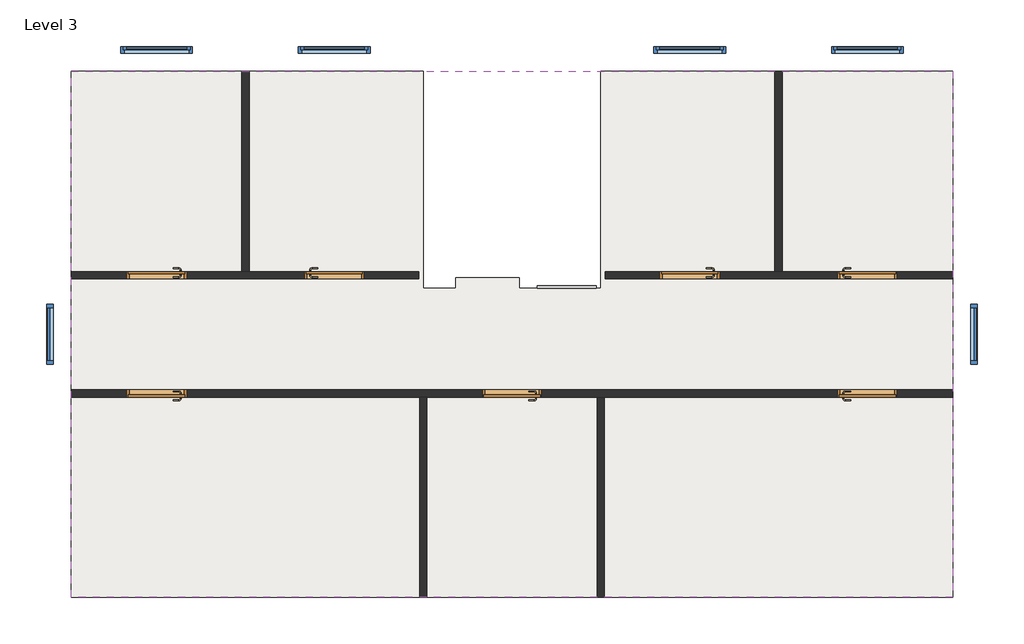
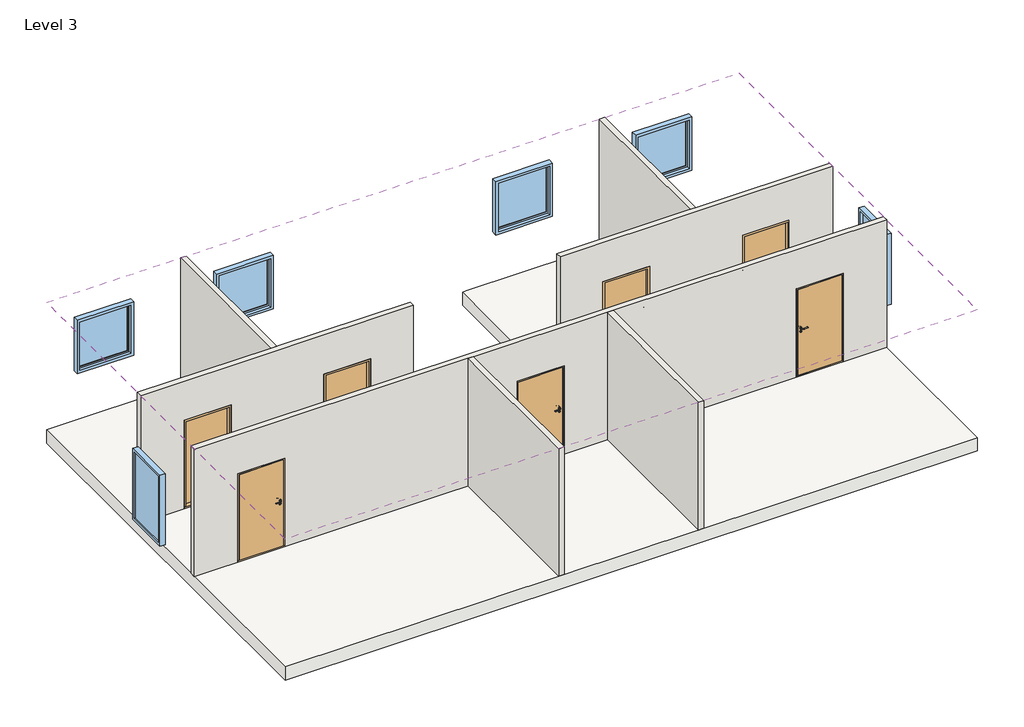
# One storey: 7 doors, 7 walls, 6 windows, 1 railing, 1 roof, 1 slab.
"""IFC4 building model written with IfcOpenShell, lengths in millimetres."""

import ifcopenshell
import ifcopenshell.guid

model = None  # the IFC model being written
_history = None  # IfcOwnerHistory: only IFC2X3 demands one
_inside = {}  # id of a spatial element -> (the spatial element, [elements in it])
_under = {}  # id of a project, library or spatial element -> (it, [spatial elements below it])
_declared = {}  # id of a project -> (the project, [libraries it declares])
_typed = {}  # id of a type object -> (the type object, [elements of that type])
_made_of = {}  # id of a material, layer set ... -> (it, [elements and type objects made of it])


def new_model(schema):
    """Start an empty IFC model of exactly this schema.

    Asked for "IFC4X3", IfcOpenShell would pick the latest addendum, in which some entities
    have other attributes; the version numbers below select the first issue.
    IFC2X3 requires an IfcOwnerHistory on every rooted entity: one is made here for all.
    """
    global model, _history
    if schema == "IFC4X3":
        model = ifcopenshell.file(schema_version=(4, 3, 0, 0))
    else:
        model = ifcopenshell.file(schema=schema)
    _inside.clear()
    _under.clear()
    _declared.clear()
    _typed.clear()
    _made_of.clear()
    _history = None
    if model.schema == "IFC2X3":
        org = make("IfcOrganization", Name="unknown")
        user = make(
            "IfcPersonAndOrganization",
            ThePerson=make("IfcPerson", FamilyName="unknown"),
            TheOrganization=org,
        )
        app = make(
            "IfcApplication",
            ApplicationDeveloper=org,
            Version="unknown",
            ApplicationFullName="unknown",
            ApplicationIdentifier="unknown",
        )
        _history = make(
            "IfcOwnerHistory",
            OwningUser=user,
            OwningApplication=app,
            ChangeAction="ADDED",
            CreationDate=0,
        )
    return model


def make(cls, **values):
    """One entity of the class cls with the attributes given. An attribute that is None is left unset."""
    return model.create_entity(
        cls, **{name: value for name, value in values.items() if value is not None}
    )


def rooted(cls, **values):
    """An entity with a GlobalId (a new one), such as an element, a storey or a relation."""
    return make(cls, GlobalId=ifcopenshell.guid.new(), OwnerHistory=_history, **values)


def si_unit(unit_type, name, prefix=None):
    """IfcSIUnit, for example si_unit("LENGTHUNIT", "METRE", prefix="MILLI")."""
    return make("IfcSIUnit", UnitType=unit_type, Prefix=prefix, Name=name)


def assignment(units):
    """IfcUnitAssignment: the units of a project."""
    return None if units is None else make("IfcUnitAssignment", Units=units)


def point(xyz):
    """IfcCartesianPoint."""
    return None if xyz is None else make("IfcCartesianPoint", Coordinates=xyz)


def direction(xyz):
    """IfcDirection."""
    return None if xyz is None else make("IfcDirection", DirectionRatios=xyz)


def frame(location, z_axis=None, x_axis=None):
    """IfcAxis2Placement3D, a coordinate frame: its origin and axes. An axis left out is left unset."""
    return make(
        "IfcAxis2Placement3D",
        Location=point(location),
        Axis=direction(z_axis),
        RefDirection=direction(x_axis),
    )


def frame_2d(location, x_axis=None):
    """IfcAxis2Placement2D, a coordinate frame in the plane: its origin and x axis."""
    return make(
        "IfcAxis2Placement2D", Location=point(location), RefDirection=direction(x_axis)
    )


def origin():
    """The frame at (0, 0, 0) with its axes left unset."""
    return frame((0.0, 0.0, 0.0))


def place(relative_to, where):
    """IfcLocalPlacement: puts the frame where relative to a parent placement (None: the world)."""
    return make(
        "IfcLocalPlacement", PlacementRelTo=relative_to, RelativePlacement=where
    )


def context(
    kind, dimensions, precision=None, world=None, true_north=None, identifier=None
):
    """IfcGeometricRepresentationContext, for example the 3D "Model" context."""
    return make(
        "IfcGeometricRepresentationContext",
        ContextIdentifier=identifier,
        ContextType=kind,
        CoordinateSpaceDimension=dimensions,
        Precision=precision,
        WorldCoordinateSystem=world,
        TrueNorth=true_north,
    )


def project(units=None, contexts=None):
    """IfcProject with its units and contexts."""
    return rooted(
        "IfcProject",
        Name="project",
        RepresentationContexts=contexts,
        UnitsInContext=assignment(units),
    )


def spatial(cls, under=None, at=None, **own):
    """A site, building, storey or space (cls), placed at a placement, below another one or the project."""
    s = rooted(cls, ObjectPlacement=at, **own)
    if under is not None:
        _under.setdefault(under.id(), (under, []))[1].append(s)
    return s


def polyline(points):
    """IfcPolyline through the points."""
    return make("IfcPolyline", Points=[point(p) for p in points])


def circle_curve(where, radius):
    """IfcCircle in the frame where."""
    return make("IfcCircle", Position=where, Radius=radius)


def ellipse_curve(where, semi_axis1, semi_axis2):
    """IfcEllipse in the frame where."""
    return make(
        "IfcEllipse", Position=where, SemiAxis1=semi_axis1, SemiAxis2=semi_axis2
    )


def trimmed(basis, trim1, trim2, sense, master):
    """IfcTrimmedCurve: the piece of a basis curve between two trims."""
    return make(
        "IfcTrimmedCurve",
        BasisCurve=basis,
        Trim1=trim1,
        Trim2=trim2,
        SenseAgreement=sense,
        MasterRepresentation=master,
    )


def segment(curve, same_sense, transition):
    """IfcCompositeCurveSegment."""
    return make(
        "IfcCompositeCurveSegment",
        Transition=transition,
        SameSense=same_sense,
        ParentCurve=curve,
    )


def composite_curve(segments, self_intersect=None):
    """IfcCompositeCurve: segments joined end to end."""
    return make("IfcCompositeCurve", Segments=segments, SelfIntersect=self_intersect)


def outline(outer, holes=None, kind="AREA"):
    """IfcArbitraryClosedProfileDef: a profile drawn as a closed curve; with holes, ...WithVoids."""
    if holes is None:
        return make("IfcArbitraryClosedProfileDef", ProfileType=kind, OuterCurve=outer)
    return make(
        "IfcArbitraryProfileDefWithVoids",
        ProfileType=kind,
        OuterCurve=outer,
        InnerCurves=holes,
    )


def extrude(swept, where, along, depth):
    """IfcExtrudedAreaSolid: the profile swept, set in the frame where, extruded along a direction by depth."""
    return make(
        "IfcExtrudedAreaSolid",
        SweptArea=swept,
        Position=where,
        ExtrudedDirection=direction(along),
        Depth=depth,
    )


def faces_of(points, faces, orient=None, outer=None):
    """IfcFace entities. A face is a list of loops; a loop is a list of indices into points, from 0.

    orient and outer hold one flag for each loop. By default every Orientation is true, the
    first loop of a face is its IfcFaceOuterBound and the others are IfcFaceBound.
    """
    made = []
    for i, loops in enumerate(faces):
        bounds = []
        for j, loop in enumerate(loops):
            is_outer = j == 0 if outer is None else outer[i][j]
            bounds.append(
                make(
                    "IfcFaceOuterBound" if is_outer else "IfcFaceBound",
                    Bound=make("IfcPolyLoop", Polygon=[points[k] for k in loop]),
                    Orientation=True if orient is None else orient[i][j],
                )
            )
        made.append(make("IfcFace", Bounds=bounds))
    return made


def faceted_brep(points, faces, orient=None, outer=None, voids=None):
    """IfcFacetedBrep: a solid bounded by flat faces; with voids (closed shells), ...WithVoids."""
    shared = [point(p) for p in points]
    hull = make("IfcClosedShell", CfsFaces=faces_of(shared, faces, orient, outer))
    if voids is None:
        return make("IfcFacetedBrep", Outer=hull)
    return make(
        "IfcFacetedBrepWithVoids",
        Outer=hull,
        Voids=[
            make(cls, CfsFaces=faces_of(shared, fs, o, b)) for cls, fs, o, b in voids
        ],
    )


def shape(context_of_items, identifier, shape_type, items):
    """IfcShapeRepresentation: the items that make up one representation, for example the "Body"."""
    return make(
        "IfcShapeRepresentation",
        ContextOfItems=context_of_items,
        RepresentationIdentifier=identifier,
        RepresentationType=shape_type,
        Items=items,
    )


def source(mapping_origin, context_of_items, identifier, shape_type, items):
    """IfcRepresentationMap: a shape defined once, which mapped items show again and again."""
    return make(
        "IfcRepresentationMap",
        MappingOrigin=mapping_origin,
        MappedRepresentation=shape(context_of_items, identifier, shape_type, items),
    )


def transform(
    local_origin,
    x_axis=None,
    y_axis=None,
    z_axis=None,
    scale=None,
    scale2=None,
    scale3=None,
    uniform=True,
):
    """IfcCartesianTransformationOperator3D, or its non-uniform kind. x_axis, y_axis, z_axis: its Axis1, 2, 3."""
    if uniform:
        return make(
            "IfcCartesianTransformationOperator3D",
            Axis1=direction(x_axis),
            Axis2=direction(y_axis),
            LocalOrigin=point(local_origin),
            Scale=scale,
            Axis3=direction(z_axis),
        )
    return make(
        "IfcCartesianTransformationOperator3DnonUniform",
        Axis1=direction(x_axis),
        Axis2=direction(y_axis),
        LocalOrigin=point(local_origin),
        Scale=scale,
        Axis3=direction(z_axis),
        Scale2=scale2,
        Scale3=scale3,
    )


def mapped(mapping_source, mapping_target):
    """IfcMappedItem: shows the shape of a source again, moved by a transform."""
    return make(
        "IfcMappedItem", MappingSource=mapping_source, MappingTarget=mapping_target
    )


def made_of(thing, what):
    """Note that an element or type object is made of a material, layer set ...; save() writes the relation."""
    if what is not None:
        _made_of.setdefault(what.id(), (what, []))[1].append(thing)
    return thing


def element(
    cls,
    number,
    at=None,
    inside=None,
    cuts=None,
    type_object=None,
    material=None,
    context=None,
    identifier="Body",
    shape_type=None,
    held_by="IfcProductDefinitionShape",
    body=None,
    shapes=None,
    **own,
):
    """One element of the class cls, such as IfcWall. Its Tag is "e" and its number.

    at: its placement. inside: the storey or other place that contains it. cuts: it is an
    opening in that element (IfcRelVoidsElement). A single representation is given by context,
    identifier, shape_type and body (its items); several are given by shapes. held_by: the class
    of the entity that holds the representations. save() writes the other relations.
    """
    e = rooted(cls, Tag="e%d" % number, ObjectPlacement=at, **own)
    if body is not None:
        shapes = [shape(context, identifier, shape_type, body)]
    if shapes is not None:
        e.Representation = make(held_by, Representations=shapes)
    if inside is not None:
        _inside.setdefault(inside.id(), (inside, []))[1].append(e)
    if cuts is not None:
        rooted(
            "IfcRelVoidsElement", RelatingBuildingElement=cuts, RelatedOpeningElement=e
        )
    if type_object is not None:
        _typed.setdefault(type_object.id(), (type_object, []))[1].append(e)
    return made_of(e, material)


def aggregate(whole, parts):
    """IfcRelAggregates: a whole, such as a stair, and the parts it consists of."""
    return rooted("IfcRelAggregates", RelatingObject=whole, RelatedObjects=parts)


def save(model, path):
    """Write the relations noted so far, then the file.

    IfcRelAggregates (storeys below a building ...), IfcRelContainedInSpatialStructure (elements
    in a storey), IfcRelDefinesByType, IfcRelAssociatesMaterial and IfcRelDeclares: one each for
    every whole, place, type object, material and project.
    """
    for whole, parts in _under.values():
        aggregate(whole, parts)
    for where, things in _inside.values():
        rooted(
            "IfcRelContainedInSpatialStructure",
            RelatedElements=things,
            RelatingStructure=where,
        )
    for kind, things in _typed.values():
        rooted("IfcRelDefinesByType", RelatedObjects=things, RelatingType=kind)
    for what, things in _made_of.values():
        rooted("IfcRelAssociatesMaterial", RelatedObjects=things, RelatingMaterial=what)
    for by, libraries in _declared.values():
        rooted("IfcRelDeclares", RelatingContext=by, RelatedDefinitions=libraries)
    model.write(path)


def plane_surface(at):
    """IfcPlane: the flat surface through the origin of the frame at, square to its z axis."""
    return make("IfcPlane", Position=at)


def cylinder_surface(at, radius):
    """IfcCylindricalSurface: all points at the distance radius from the z axis of the frame at."""
    return make("IfcCylindricalSurface", Position=at, Radius=radius)


def revolved_surface(curve, axis_point, axis_direction):
    """IfcSurfaceOfRevolution: the curve turned about the line through axis_point along axis_direction."""
    return make(
        "IfcSurfaceOfRevolution",
        SweptCurve=make("IfcArbitraryOpenProfileDef", ProfileType="CURVE", Curve=curve),
        AxisPosition=make("IfcAxis1Placement", Location=point(axis_point), Axis=direction(axis_direction)),
    )


def advanced_brep(points, edges, surfaces, faces):
    """IfcAdvancedBrep: a solid bounded by faces that lie on surfaces and meet in shared edges.

    An edge is (start, end): straight between two places in points (the first is 0);
    or (start, end, curve); or (start, end, curve, False) where it runs against its curve.
    A face is (place in surfaces, loops), or (place, loops, False) where it looks against
    its surface's normal. A loop lists edges by number (the first is 1), with a minus sign
    where the edge is run from its end to its start. The first loop is the outer one.
    """
    corners = [point(p) for p in points]
    vertices = [make("IfcVertexPoint", VertexGeometry=c) for c in corners]
    made = []
    for start, end, *more in edges:
        made.append(
            make(
                "IfcEdgeCurve",
                EdgeStart=vertices[start],
                EdgeEnd=vertices[end],
                EdgeGeometry=more[0] if more else make("IfcPolyline", Points=[corners[start], corners[end]]),
                SameSense=more[1] if len(more) > 1 else True,
            )
        )
    hull = []
    for where, loops, *sense in faces:
        bounds = []
        for j, loop in enumerate(loops):
            ring = [make("IfcOrientedEdge", EdgeElement=made[abs(k) - 1], Orientation=k > 0) for k in loop]
            bounds.append(
                make(
                    "IfcFaceOuterBound" if j == 0 else "IfcFaceBound",
                    Bound=make("IfcEdgeLoop", EdgeList=ring),
                    Orientation=True,
                )
            )
        hull.append(make("IfcAdvancedFace", Bounds=bounds, FaceSurface=surfaces[where], SameSense=sense[0] if sense else True))
    return make("IfcAdvancedBrep", Outer=make("IfcClosedShell", CfsFaces=hull))


def int_single_flush_10x20m_e84bf50b(model_context):
    return source(origin(), model_context, "Body", "SolidModel", [
        extrude(outline(composite_curve([segment(trimmed(circle_curve(frame_2d((1090.0, -406.0)), 20.0), [point((1070.0, -406.0))], [point((1110.0, -406.0))], False, "CARTESIAN"), True, "CONTINUOUS"), segment(trimmed(circle_curve(frame_2d((1090.0, -406.0)), 20.0), [point((1110.0, -406.0))], [point((1070.0, -406.0))], False, "CARTESIAN"), True, "CONTINUOUS")], self_intersect=False)), frame((0.0, 60.0, 0.0), z_axis=(0.0, 1.0, 0.0), x_axis=(0.0, 0.0, 1.0)), (0.0, 0.0, 1.0), 2.0),
        advanced_brep(
        [(-413.5, 62.0, 1090.0), (-398.5, 62.0, 1090.0), (-413.5, 84.5, 1090.0), (-398.5, 84.5, 1090.0), (-376.0, 107.0, 1090.0), (-376.0, 122.0, 1090.0), (-281.0, 122.0, 1090.0), (-281.0, 107.0, 1090.0)],
        [
            (0, 1, circle_curve(frame((-406.0, 62.0, 1090.0), z_axis=(0.0, -1.0, 0.0), x_axis=(1.0, 0.0, 0.0)), 7.5)),
            (1, 0, circle_curve(frame((-406.0, 62.0, 1090.0), z_axis=(0.0, -1.0, 0.0), x_axis=(1.0, 0.0, 0.0)), 7.5)),
            (0, 2),
            (2, 3, circle_curve(frame((-406.0, 84.5, 1090.0), z_axis=(0.0, -1.0, 0.0), x_axis=(1.0, 0.0, 0.0)), 7.5)),
            (3, 1),
            (3, 2, circle_curve(frame((-406.0, 84.5, 1090.0), z_axis=(0.0, -1.0, 0.0), x_axis=(1.0, 0.0, 0.0)), 7.5)),
            (4, 3, circle_curve(frame((-376.0, 84.5, 1090.0), z_axis=(0.0, 0.0, 1.0), x_axis=(-1.0, 0.0, 0.0)), 22.5)),
            (2, 5, circle_curve(frame((-376.0, 84.5, 1090.0), z_axis=(0.0, 0.0, -1.0), x_axis=(-1.0, 0.0, 0.0)), 37.5)),
            (5, 4, circle_curve(frame((-376.0, 114.5, 1090.0), z_axis=(-1.0, 0.0, 0.0), x_axis=(0.0, -1.0, 0.0)), 7.5)),
            (4, 5, circle_curve(frame((-376.0, 114.5, 1090.0), z_axis=(-1.0, 0.0, 0.0), x_axis=(0.0, -1.0, 0.0)), 7.5)),
            (5, 6),
            (6, 7, circle_curve(frame((-281.0, 114.5, 1090.0), z_axis=(-1.0, 0.0, 0.0), x_axis=(0.0, -1.0, 0.0)), 7.5)),
            (7, 4),
            (7, 6, circle_curve(frame((-281.0, 114.5, 1090.0), z_axis=(-1.0, 0.0, 0.0), x_axis=(0.0, -1.0, 0.0)), 7.5)),
        ],
        [
            plane_surface(frame((-406.0, 62.0, 1090.0), z_axis=(0.0, -1.0, 0.0), x_axis=(0.0, 0.0, -1.0))),
            cylinder_surface(frame((-406.0, 62.0, 1090.0), z_axis=(0.0, -1.0, 0.0), x_axis=(1.0, 0.0, 0.0)), 7.5),
            revolved_surface(trimmed(ellipse_curve(frame((-406.0, 84.5, 1090.0), z_axis=(0.0, -1.0, 0.0), x_axis=(1.0, 0.0, 0.0)), 7.5, 7.5), [point((-413.5, 84.5, 1090.0))], [point((-398.5, 84.5, 1090.0))], True, "CARTESIAN"), (-376.0, 84.5, 1090.0), (0.0, 0.0, -1.0)),
            revolved_surface(trimmed(ellipse_curve(frame((-406.0, 84.5, 1090.0), z_axis=(0.0, -1.0, 0.0), x_axis=(1.0, 0.0, 0.0)), 7.5, 7.5), [point((-398.5, 84.5, 1090.0))], [point((-413.5, 84.5, 1090.0))], True, "CARTESIAN"), (-376.0, 84.5, 1090.0), (0.0, 0.0, -1.0)),
            cylinder_surface(frame((-376.0, 114.5, 1090.0), z_axis=(-1.0, 0.0, 0.0), x_axis=(0.0, -1.0, 0.0)), 7.5),
            plane_surface(frame((-281.0, 114.5, 1090.0), z_axis=(1.0, 0.0, 0.0), x_axis=(0.0, 0.0, -1.0))),
        ],
        [
            (0, [[1, 2]]),
            (1, [[-1, 3, 4, 5]]),
            (1, [[-2, -5, 6, -3]]),
            (2, [[7, -4, 8, 9]]),
            (3, [[-8, -6, -7, 10]]),
            (4, [[-9, 11, 12, 13]]),
            (4, [[-10, -13, 14, -11]]),
            (5, [[-14, -12]]),
        ],
    ),
        extrude(outline(composite_curve([segment(trimmed(circle_curve(frame_2d((1010.0, -406.0)), 20.0), [point((990.0, -406.0))], [point((1030.0, -406.0))], False, "CARTESIAN"), True, "CONTINUOUS"), segment(trimmed(circle_curve(frame_2d((1010.0, -406.0)), 20.0), [point((1030.0, -406.0))], [point((990.0, -406.0))], False, "CARTESIAN"), True, "CONTINUOUS")], self_intersect=False), holes=[composite_curve([segment(trimmed(circle_curve(frame_2d((1015.0, -406.0)), 3.0), [point((1012.4019238, -407.5))], [point((1012.4019238, -404.5))], True, "CARTESIAN"), True, "CONTINUOUS"), segment(polyline([(1012.4019238, -404.5), (1000.0, -404.5), (1000.0, -407.5), (1012.4019238, -407.5)]), True, "CONTINUOUS")], self_intersect=False)]), frame((0.0, 60.0, 0.0), z_axis=(0.0, 1.0, 0.0), x_axis=(0.0, 0.0, 1.0)), (0.0, 0.0, 1.0), 2.0),
        extrude(outline(composite_curve([segment(trimmed(circle_curve(frame_2d((1090.0, -406.0)), 20.0), [point((1070.0, -406.0))], [point((1110.0, -406.0))], False, "CARTESIAN"), True, "CONTINUOUS"), segment(trimmed(circle_curve(frame_2d((1090.0, -406.0)), 20.0), [point((1110.0, -406.0))], [point((1070.0, -406.0))], False, "CARTESIAN"), True, "CONTINUOUS")], self_intersect=False)), frame((0.0, 18.0, 0.0), z_axis=(0.0, 1.0, 0.0), x_axis=(0.0, 0.0, 1.0)), (0.0, 0.0, 1.0), 2.0),
        advanced_brep(
        [(-413.5, 18.0, 1090.0), (-398.5, 18.0, 1090.0), (-398.5, -4.5, 1090.0), (-413.5, -4.5, 1090.0), (-376.0, -27.0, 1090.0), (-376.0, -42.0, 1090.0), (-281.0, -27.0, 1090.0), (-281.0, -42.0, 1090.0)],
        [
            (0, 1, circle_curve(frame((-406.0, 18.0, 1090.0), z_axis=(0.0, 1.0, 0.0), x_axis=(1.0, 0.0, 0.0)), 7.5)),
            (1, 0, circle_curve(frame((-406.0, 18.0, 1090.0), z_axis=(0.0, 1.0, 0.0), x_axis=(1.0, 0.0, 0.0)), 7.5)),
            (1, 2),
            (2, 3, circle_curve(frame((-406.0, -4.5, 1090.0), z_axis=(0.0, 1.0, 0.0), x_axis=(1.0, 0.0, 0.0)), 7.5)),
            (3, 0),
            (3, 2, circle_curve(frame((-406.0, -4.5, 1090.0), z_axis=(0.0, 1.0, 0.0), x_axis=(1.0, 0.0, 0.0)), 7.5)),
            (4, 5, circle_curve(frame((-376.0, -34.5, 1090.0), z_axis=(-1.0, 0.0, 0.0), x_axis=(0.0, 1.0, 0.0)), 7.5)),
            (5, 3, circle_curve(frame((-376.0, -4.5, 1090.0), z_axis=(0.0, 0.0, -1.0), x_axis=(-1.0, 0.0, 0.0)), 37.5)),
            (2, 4, circle_curve(frame((-376.0, -4.5, 1090.0), z_axis=(0.0, 0.0, 1.0), x_axis=(-1.0, 0.0, 0.0)), 22.5)),
            (5, 4, circle_curve(frame((-376.0, -34.5, 1090.0), z_axis=(-1.0, 0.0, 0.0), x_axis=(0.0, 1.0, 0.0)), 7.5)),
            (4, 6),
            (6, 7, circle_curve(frame((-281.0, -34.5, 1090.0), z_axis=(-1.0, 0.0, 0.0), x_axis=(0.0, 1.0, 0.0)), 7.5)),
            (7, 5),
            (7, 6, circle_curve(frame((-281.0, -34.5, 1090.0), z_axis=(-1.0, 0.0, 0.0), x_axis=(0.0, 1.0, 0.0)), 7.5)),
        ],
        [
            plane_surface(frame((-406.0, 18.0, 1090.0), z_axis=(0.0, 1.0, 0.0), x_axis=(0.0, 0.0, -1.0))),
            cylinder_surface(frame((-406.0, 18.0, 1090.0), z_axis=(0.0, 1.0, 0.0), x_axis=(1.0, 0.0, 0.0)), 7.5),
            revolved_surface(trimmed(ellipse_curve(frame((-406.0, -4.5, 1090.0), z_axis=(0.0, -1.0, 0.0), x_axis=(1.0, 0.0, 0.0)), 7.5, 7.5), [point((-413.5, -4.5, 1090.0))], [point((-398.5, -4.5, 1090.0))], True, "CARTESIAN"), (-376.0, -4.5, 1090.0), (0.0, 0.0, -1.0)),
            revolved_surface(trimmed(ellipse_curve(frame((-406.0, -4.5, 1090.0), z_axis=(0.0, -1.0, 0.0), x_axis=(1.0, 0.0, 0.0)), 7.5, 7.5), [point((-398.5, -4.5, 1090.0))], [point((-413.5, -4.5, 1090.0))], True, "CARTESIAN"), (-376.0, -4.5, 1090.0), (0.0, 0.0, -1.0)),
            cylinder_surface(frame((-376.0, -34.5, 1090.0), z_axis=(-1.0, 0.0, 0.0), x_axis=(0.0, 1.0, 0.0)), 7.5),
            plane_surface(frame((-281.0, -34.5, 1090.0), z_axis=(1.0, 0.0, 0.0), x_axis=(0.0, 0.0, -1.0))),
        ],
        [
            (0, [[1, 2]]),
            (1, [[3, 4, 5, -2]]),
            (1, [[-5, 6, -3, -1]]),
            (2, [[7, 8, -4, 9]]),
            (3, [[10, -9, -6, -8]]),
            (4, [[11, 12, 13, -7]]),
            (4, [[-13, 14, -11, -10]]),
            (5, [[-12, -14]]),
        ],
    ),
        extrude(outline(composite_curve([segment(trimmed(circle_curve(frame_2d((1010.0, -406.0)), 20.0), [point((990.0, -406.0))], [point((1030.0, -406.0))], False, "CARTESIAN"), True, "CONTINUOUS"), segment(trimmed(circle_curve(frame_2d((1010.0, -406.0)), 20.0), [point((1030.0, -406.0))], [point((990.0, -406.0))], False, "CARTESIAN"), True, "CONTINUOUS")], self_intersect=False), holes=[composite_curve([segment(trimmed(circle_curve(frame_2d((1015.0, -406.0)), 3.0), [point((1012.4019238, -407.5))], [point((1012.4019238, -404.5))], True, "CARTESIAN"), True, "CONTINUOUS"), segment(polyline([(1012.4019238, -404.5), (1000.0, -404.5), (1000.0, -407.5), (1012.4019238, -407.5)]), True, "CONTINUOUS")], self_intersect=False)]), frame((0.0, 18.0, 0.0), z_axis=(0.0, 1.0, 0.0), x_axis=(0.0, 0.0, 1.0)), (0.0, 0.0, 1.0), 2.0),
        extrude(outline(polyline([(476.0, 20.0), (-476.0, 20.0), (-476.0, 60.0), (476.0, 60.0), (476.0, 20.0)])), frame((0.0, 0.0, 30.0), z_axis=(0.0, 0.0, 1.0), x_axis=(1.0, 0.0, 0.0)), (0.0, 0.0, 1.0), 1952.0),
        extrude(outline(polyline([(20.0, 42.0), (20.0, 30.0), (60.0, 30.0), (60.0, 0.0), (-60.0, 0.0), (-60.0, 42.0), (20.0, 42.0)])), frame((-506.0, 0.0, 0.0), z_axis=(1.0, 0.0, 0.0), x_axis=(0.0, 1.0, 0.0)), (0.0, 0.0, 1.0), 1012.0),
        faceted_brep([(-476.0, 20.0, 1982.0), (476.0, 20.0, 1982.0), (476.0, 20.0, 42.0), (464.0, 20.0, 42.0), (464.0, 20.0, 1970.0), (-464.0, 20.0, 1970.0), (-464.0, 20.0, 42.0), (-476.0, 20.0, 42.0), (-476.0, 60.0, 1982.0), (-476.0, 20.0, 30.0), (-476.0, 60.0, 30.0), (-506.0, 20.0, 42.0), (-506.0, 20.0, 30.0), (506.0, 20.0, 42.0), (476.0, 20.0, 30.0), (506.0, 20.0, 30.0), (-506.0, 60.0, 30.0), (476.0, 60.0, 30.0), (506.0, 60.0, 30.0), (-506.0, 60.0, 2012.0), (506.0, 60.0, 2012.0), (476.0, 60.0, 1982.0), (-464.0, -60.0, 42.0), (-506.0, -60.0, 42.0), (506.0, -60.0, 42.0), (464.0, -60.0, 42.0), (464.0, -60.0, 1970.0), (-464.0, -60.0, 1970.0), (506.0, -60.0, 2012.0), (-506.0, -60.0, 2012.0)], [[[0, 1, 2, 3, 4, 5, 6, 7]], [[8, 0, 7, 9, 10]], [[7, 11, 12, 9]], [[13, 2, 14, 15]], [[9, 12, 16, 10]], [[15, 14, 17, 18]], [[19, 20, 18, 17, 21, 8, 10, 16]], [[1, 21, 17, 14, 2]], [[11, 7, 6, 22, 23]], [[2, 13, 24, 25, 3]], [[26, 4, 3, 25]], [[5, 27, 22, 6]], [[27, 26, 25, 24, 28, 29, 23, 22]], [[20, 28, 24, 13, 15, 18]], [[29, 19, 16, 12, 11, 23]], [[0, 8, 21, 1]], [[5, 4, 26, 27]], [[29, 28, 20, 19]]]),
    ])


def int_single_flush_10x20m_68751a9d(model_context):
    return source(origin(), model_context, "Body", "SolidModel", [
        extrude(outline(composite_curve([segment(trimmed(circle_curve(frame_2d((1090.0, -406.0)), 20.0), [point((1070.0, -406.0))], [point((1110.0, -406.0))], False, "CARTESIAN"), True, "CONTINUOUS"), segment(trimmed(circle_curve(frame_2d((1090.0, -406.0)), 20.0), [point((1110.0, -406.0))], [point((1070.0, -406.0))], False, "CARTESIAN"), True, "CONTINUOUS")], self_intersect=False)), frame((0.0, -62.0, 0.0), z_axis=(0.0, 1.0, 0.0), x_axis=(0.0, 0.0, 1.0)), (0.0, 0.0, 1.0), 2.0),
        advanced_brep(
        [(-413.5, -62.0, 1090.0), (-398.5, -62.0, 1090.0), (-398.5, -84.5, 1090.0), (-413.5, -84.5, 1090.0), (-376.0, -107.0, 1090.0), (-376.0, -122.0, 1090.0), (-281.0, -107.0, 1090.0), (-281.0, -122.0, 1090.0)],
        [
            (0, 1, circle_curve(frame((-406.0, -62.0, 1090.0), z_axis=(0.0, 1.0, 0.0), x_axis=(1.0, 0.0, 0.0)), 7.5)),
            (1, 0, circle_curve(frame((-406.0, -62.0, 1090.0), z_axis=(0.0, 1.0, 0.0), x_axis=(1.0, 0.0, 0.0)), 7.5)),
            (1, 2),
            (2, 3, circle_curve(frame((-406.0, -84.5, 1090.0), z_axis=(0.0, 1.0, 0.0), x_axis=(1.0, 0.0, 0.0)), 7.5)),
            (3, 0),
            (3, 2, circle_curve(frame((-406.0, -84.5, 1090.0), z_axis=(0.0, 1.0, 0.0), x_axis=(1.0, 0.0, 0.0)), 7.5)),
            (4, 5, circle_curve(frame((-376.0, -114.5, 1090.0), z_axis=(-1.0, 0.0, 0.0), x_axis=(0.0, 1.0, 0.0)), 7.5)),
            (5, 3, circle_curve(frame((-376.0, -84.5, 1090.0), z_axis=(0.0, 0.0, -1.0), x_axis=(-1.0, 0.0, 0.0)), 37.5)),
            (2, 4, circle_curve(frame((-376.0, -84.5, 1090.0), z_axis=(0.0, 0.0, 1.0), x_axis=(-1.0, 0.0, 0.0)), 22.5)),
            (5, 4, circle_curve(frame((-376.0, -114.5, 1090.0), z_axis=(-1.0, 0.0, 0.0), x_axis=(0.0, 1.0, 0.0)), 7.5)),
            (4, 6),
            (6, 7, circle_curve(frame((-281.0, -114.5, 1090.0), z_axis=(-1.0, 0.0, 0.0), x_axis=(0.0, 1.0, 0.0)), 7.5)),
            (7, 5),
            (7, 6, circle_curve(frame((-281.0, -114.5, 1090.0), z_axis=(-1.0, 0.0, 0.0), x_axis=(0.0, 1.0, 0.0)), 7.5)),
        ],
        [
            plane_surface(frame((-406.0, -62.0, 1090.0), z_axis=(0.0, 1.0, 0.0), x_axis=(0.0, 0.0, -1.0))),
            cylinder_surface(frame((-406.0, -62.0, 1090.0), z_axis=(0.0, 1.0, 0.0), x_axis=(1.0, 0.0, 0.0)), 7.5),
            revolved_surface(trimmed(ellipse_curve(frame((-406.0, -84.5, 1090.0), z_axis=(0.0, -1.0, 0.0), x_axis=(1.0, 0.0, 0.0)), 7.5, 7.5), [point((-413.5, -84.5, 1090.0))], [point((-398.5, -84.5, 1090.0))], True, "CARTESIAN"), (-376.0, -84.5, 1090.0), (0.0, 0.0, -1.0)),
            revolved_surface(trimmed(ellipse_curve(frame((-406.0, -84.5, 1090.0), z_axis=(0.0, -1.0, 0.0), x_axis=(1.0, 0.0, 0.0)), 7.5, 7.5), [point((-398.5, -84.5, 1090.0))], [point((-413.5, -84.5, 1090.0))], True, "CARTESIAN"), (-376.0, -84.5, 1090.0), (0.0, 0.0, -1.0)),
            cylinder_surface(frame((-376.0, -114.5, 1090.0), z_axis=(-1.0, 0.0, 0.0), x_axis=(0.0, 1.0, 0.0)), 7.5),
            plane_surface(frame((-281.0, -114.5, 1090.0), z_axis=(1.0, 0.0, 0.0), x_axis=(0.0, 0.0, -1.0))),
        ],
        [
            (0, [[1, 2]]),
            (1, [[3, 4, 5, -2]]),
            (1, [[-5, 6, -3, -1]]),
            (2, [[7, 8, -4, 9]]),
            (3, [[10, -9, -6, -8]]),
            (4, [[11, 12, 13, -7]]),
            (4, [[-13, 14, -11, -10]]),
            (5, [[-12, -14]]),
        ],
    ),
        extrude(outline(composite_curve([segment(trimmed(circle_curve(frame_2d((1010.0, -406.0)), 20.0), [point((990.0, -406.0))], [point((1030.0, -406.0))], False, "CARTESIAN"), True, "CONTINUOUS"), segment(trimmed(circle_curve(frame_2d((1010.0, -406.0)), 20.0), [point((1030.0, -406.0))], [point((990.0, -406.0))], False, "CARTESIAN"), True, "CONTINUOUS")], self_intersect=False), holes=[composite_curve([segment(trimmed(circle_curve(frame_2d((1015.0, -406.0)), 3.0), [point((1012.4019238, -407.5))], [point((1012.4019238, -404.5))], True, "CARTESIAN"), True, "CONTINUOUS"), segment(polyline([(1012.4019238, -404.5), (1000.0, -404.5), (1000.0, -407.5), (1012.4019238, -407.5)]), True, "CONTINUOUS")], self_intersect=False)]), frame((0.0, -62.0, 0.0), z_axis=(0.0, 1.0, 0.0), x_axis=(0.0, 0.0, 1.0)), (0.0, 0.0, 1.0), 2.0),
        extrude(outline(composite_curve([segment(trimmed(circle_curve(frame_2d((1090.0, -406.0)), 20.0), [point((1070.0, -406.0))], [point((1110.0, -406.0))], False, "CARTESIAN"), True, "CONTINUOUS"), segment(trimmed(circle_curve(frame_2d((1090.0, -406.0)), 20.0), [point((1110.0, -406.0))], [point((1070.0, -406.0))], False, "CARTESIAN"), True, "CONTINUOUS")], self_intersect=False)), frame((0.0, -20.0, 0.0), z_axis=(0.0, 1.0, 0.0), x_axis=(0.0, 0.0, 1.0)), (0.0, 0.0, 1.0), 2.0),
        advanced_brep(
        [(-413.5, -18.0, 1090.0), (-398.5, -18.0, 1090.0), (-413.5, 4.5, 1090.0), (-398.5, 4.5, 1090.0), (-376.0, 27.0, 1090.0), (-376.0, 42.0, 1090.0), (-281.0, 42.0, 1090.0), (-281.0, 27.0, 1090.0)],
        [
            (0, 1, circle_curve(frame((-406.0, -18.0, 1090.0), z_axis=(0.0, -1.0, 0.0), x_axis=(1.0, 0.0, 0.0)), 7.5)),
            (1, 0, circle_curve(frame((-406.0, -18.0, 1090.0), z_axis=(0.0, -1.0, 0.0), x_axis=(1.0, 0.0, 0.0)), 7.5)),
            (0, 2),
            (2, 3, circle_curve(frame((-406.0, 4.5, 1090.0), z_axis=(0.0, -1.0, 0.0), x_axis=(1.0, 0.0, 0.0)), 7.5)),
            (3, 1),
            (3, 2, circle_curve(frame((-406.0, 4.5, 1090.0), z_axis=(0.0, -1.0, 0.0), x_axis=(1.0, 0.0, 0.0)), 7.5)),
            (4, 3, circle_curve(frame((-376.0, 4.5, 1090.0), z_axis=(0.0, 0.0, 1.0), x_axis=(-1.0, 0.0, 0.0)), 22.5)),
            (2, 5, circle_curve(frame((-376.0, 4.5, 1090.0), z_axis=(0.0, 0.0, -1.0), x_axis=(-1.0, 0.0, 0.0)), 37.5)),
            (5, 4, circle_curve(frame((-376.0, 34.5, 1090.0), z_axis=(-1.0, 0.0, 0.0), x_axis=(0.0, -1.0, 0.0)), 7.5)),
            (4, 5, circle_curve(frame((-376.0, 34.5, 1090.0), z_axis=(-1.0, 0.0, 0.0), x_axis=(0.0, -1.0, 0.0)), 7.5)),
            (5, 6),
            (6, 7, circle_curve(frame((-281.0, 34.5, 1090.0), z_axis=(-1.0, 0.0, 0.0), x_axis=(0.0, -1.0, 0.0)), 7.5)),
            (7, 4),
            (7, 6, circle_curve(frame((-281.0, 34.5, 1090.0), z_axis=(-1.0, 0.0, 0.0), x_axis=(0.0, -1.0, 0.0)), 7.5)),
        ],
        [
            plane_surface(frame((-406.0, -18.0, 1090.0), z_axis=(0.0, -1.0, 0.0), x_axis=(0.0, 0.0, -1.0))),
            cylinder_surface(frame((-406.0, -18.0, 1090.0), z_axis=(0.0, -1.0, 0.0), x_axis=(1.0, 0.0, 0.0)), 7.5),
            revolved_surface(trimmed(ellipse_curve(frame((-406.0, 4.5, 1090.0), z_axis=(0.0, -1.0, 0.0), x_axis=(1.0, 0.0, 0.0)), 7.5, 7.5), [point((-413.5, 4.5, 1090.0))], [point((-398.5, 4.5, 1090.0))], True, "CARTESIAN"), (-376.0, 4.5, 1090.0), (0.0, 0.0, -1.0)),
            revolved_surface(trimmed(ellipse_curve(frame((-406.0, 4.5, 1090.0), z_axis=(0.0, -1.0, 0.0), x_axis=(1.0, 0.0, 0.0)), 7.5, 7.5), [point((-398.5, 4.5, 1090.0))], [point((-413.5, 4.5, 1090.0))], True, "CARTESIAN"), (-376.0, 4.5, 1090.0), (0.0, 0.0, -1.0)),
            cylinder_surface(frame((-376.0, 34.5, 1090.0), z_axis=(-1.0, 0.0, 0.0), x_axis=(0.0, -1.0, 0.0)), 7.5),
            plane_surface(frame((-281.0, 34.5, 1090.0), z_axis=(1.0, 0.0, 0.0), x_axis=(0.0, 0.0, -1.0))),
        ],
        [
            (0, [[1, 2]]),
            (1, [[-1, 3, 4, 5]]),
            (1, [[-2, -5, 6, -3]]),
            (2, [[7, -4, 8, 9]]),
            (3, [[-8, -6, -7, 10]]),
            (4, [[-9, 11, 12, 13]]),
            (4, [[-10, -13, 14, -11]]),
            (5, [[-14, -12]]),
        ],
    ),
        extrude(outline(composite_curve([segment(trimmed(circle_curve(frame_2d((1010.0, -406.0)), 20.0), [point((990.0, -406.0))], [point((1030.0, -406.0))], False, "CARTESIAN"), True, "CONTINUOUS"), segment(trimmed(circle_curve(frame_2d((1010.0, -406.0)), 20.0), [point((1030.0, -406.0))], [point((990.0, -406.0))], False, "CARTESIAN"), True, "CONTINUOUS")], self_intersect=False), holes=[composite_curve([segment(trimmed(circle_curve(frame_2d((1015.0, -406.0)), 3.0), [point((1012.4019238, -407.5))], [point((1012.4019238, -404.5))], True, "CARTESIAN"), True, "CONTINUOUS"), segment(polyline([(1012.4019238, -404.5), (1000.0, -404.5), (1000.0, -407.5), (1012.4019238, -407.5)]), True, "CONTINUOUS")], self_intersect=False)]), frame((0.0, -20.0, 0.0), z_axis=(0.0, 1.0, 0.0), x_axis=(0.0, 0.0, 1.0)), (0.0, 0.0, 1.0), 2.0),
        extrude(outline(polyline([(476.0, -20.0), (476.0, -60.0), (-476.0, -60.0), (-476.0, -20.0), (476.0, -20.0)])), frame((0.0, 0.0, 30.0), z_axis=(0.0, 0.0, 1.0), x_axis=(1.0, 0.0, 0.0)), (0.0, 0.0, 1.0), 1952.0),
        extrude(outline(polyline([(-20.0, 42.0), (60.0, 42.0), (60.0, 0.0), (-60.0, 0.0), (-60.0, 30.0), (-20.0, 30.0), (-20.0, 42.0)])), frame((-506.0, 0.0, 0.0), z_axis=(1.0, 0.0, 0.0), x_axis=(0.0, 1.0, 0.0)), (0.0, 0.0, 1.0), 1012.0),
        faceted_brep([(-476.0, -20.0, 1982.0), (-476.0, -20.0, 42.0), (-464.0, -20.0, 42.0), (-464.0, -20.0, 1970.0), (464.0, -20.0, 1970.0), (464.0, -20.0, 42.0), (476.0, -20.0, 42.0), (476.0, -20.0, 1982.0), (-476.0, -60.0, 1982.0), (-476.0, -60.0, 30.0), (-476.0, -20.0, 30.0), (-506.0, -20.0, 30.0), (-506.0, -20.0, 42.0), (506.0, -20.0, 42.0), (506.0, -20.0, 30.0), (476.0, -20.0, 30.0), (-506.0, -60.0, 30.0), (506.0, -60.0, 30.0), (476.0, -60.0, 30.0), (-506.0, -60.0, 2012.0), (476.0, -60.0, 1982.0), (506.0, -60.0, 2012.0), (464.0, 60.0, 42.0), (506.0, 60.0, 42.0), (-506.0, 60.0, 42.0), (-464.0, 60.0, 42.0), (464.0, 60.0, 1970.0), (-464.0, 60.0, 1970.0), (-506.0, 60.0, 2012.0), (506.0, 60.0, 2012.0)], [[[0, 1, 2, 3, 4, 5, 6, 7]], [[8, 9, 10, 1, 0]], [[1, 10, 11, 12]], [[13, 14, 15, 6]], [[10, 9, 16, 11]], [[14, 17, 18, 15]], [[19, 16, 9, 8, 20, 18, 17, 21]], [[7, 6, 15, 18, 20]], [[6, 5, 22, 23, 13]], [[12, 24, 25, 2, 1]], [[26, 22, 5, 4]], [[3, 2, 25, 27]], [[27, 25, 24, 28, 29, 23, 22, 26]], [[21, 17, 14, 13, 23, 29]], [[28, 24, 12, 11, 16, 19]], [[0, 7, 20, 8]], [[3, 27, 26, 4]], [[28, 19, 21, 29]]]),
    ])


def sketch_1100mm_82aaa055(model_context):
    return source(origin(), model_context, "Body", "SweptSolid", [
        extrude(outline(composite_curve([segment(trimmed(circle_curve(frame_2d((5300.0, 7480.0)), 20.0), [point((5280.0, 7480.0))], [point((5320.0, 7480.0))], False, "CARTESIAN"), True, "CONTINUOUS"), segment(trimmed(circle_curve(frame_2d((5300.0, 7480.0)), 20.0), [point((5320.0, 7480.0))], [point((5280.0, 7480.0))], False, "CARTESIAN"), True, "CONTINUOUS")], self_intersect=False)), frame((7925.0, 0.0, 0.0), z_axis=(1.0, 0.0, 0.0), x_axis=(0.0, 1.0, 0.0)), (0.0, 0.0, 1.0), 1000.0),
    ])


def fixed_10x16m_885135a8(model_context):
    return source(origin(), model_context, "Body", "SweptSolid", [
        extrude(outline(polyline([(2412.0, 506.0), (2412.0, -506.0), (800.0, -506.0), (800.0, 506.0), (2412.0, 506.0)]), holes=[polyline([(857.0, 449.0), (857.0, -449.0), (2355.0, -449.0), (2355.0, 449.0), (857.0, 449.0)])]), frame((0.0, 69.0, 0.0), z_axis=(0.0, 1.0, 0.0), x_axis=(0.0, 0.0, 1.0)), (0.0, 0.0, 1.0), 115.0),
        extrude(outline(polyline([(-449.0, 162.0), (449.0, 162.0), (449.0, 134.0), (-449.0, 134.0), (-449.0, 162.0)])), frame((0.0, 0.0, 857.0), z_axis=(0.0, 0.0, 1.0), x_axis=(1.0, 0.0, 0.0)), (0.0, 0.0, 1.0), 1498.0),
    ])


def single_light_12x12m_8659da90(model_context):
    return source(origin(), model_context, "Body", "SolidModel", [
        extrude(outline(polyline([(1970.0, -564.0), (842.0, -564.0), (842.0, 564.0), (1970.0, 564.0), (1970.0, -564.0)]), holes=[polyline([(1920.0, 514.0), (892.0, 514.0), (892.0, -514.0), (1920.0, -514.0), (1920.0, 514.0)])]), frame((0.0, 134.0, 0.0), z_axis=(0.0, 1.0, 0.0), x_axis=(0.0, 0.0, 1.0)), (0.0, 0.0, 1.0), 50.0),
        faceted_brep([(-606.0, 69.0, 800.0), (-606.0, 184.0, 800.0), (606.0, 184.0, 800.0), (606.0, 69.0, 800.0), (606.0, 184.0, 2012.0), (606.0, 69.0, 2012.0), (-606.0, 184.0, 2012.0), (564.0, 184.0, 1970.0), (-564.0, 184.0, 1970.0), (-564.0, 184.0, 842.0), (564.0, 184.0, 842.0), (-606.0, 69.0, 2012.0), (549.0, 69.0, 857.0), (-549.0, 69.0, 857.0), (-549.0, 69.0, 1955.0), (549.0, 69.0, 1955.0), (-549.0, 134.0, 857.0), (549.0, 134.0, 857.0), (549.0, 134.0, 1955.0), (564.0, 134.0, 842.0), (-564.0, 134.0, 842.0), (-564.0, 134.0, 1970.0), (564.0, 134.0, 1970.0), (-549.0, 134.0, 1955.0)], [[[0, 1, 2, 3]], [[3, 2, 4, 5]], [[2, 1, 6, 4], [7, 8, 9, 10]], [[5, 11, 0, 3], [12, 13, 14, 15]], [[16, 13, 12, 17]], [[17, 12, 15, 18]], [[19, 20, 21, 22], [18, 23, 16, 17]], [[9, 20, 19, 10]], [[10, 19, 22, 7]], [[11, 6, 1, 0]], [[23, 14, 13, 16]], [[8, 21, 20, 9]], [[5, 4, 6, 11]], [[18, 15, 14, 23]], [[7, 22, 21, 8]]]),
        extrude(outline(polyline([(-514.0, 170.0), (514.0, 170.0), (514.0, 148.0), (-514.0, 148.0), (-514.0, 170.0)])), frame((0.0, 0.0, 892.0), z_axis=(0.0, 0.0, 1.0), x_axis=(1.0, 0.0, 0.0)), (0.0, 0.0, 1.0), 1028.0),
    ])


model = new_model("IFC4")

# Units and contexts
model_context = context("Model", 3, world=origin())
ifc_project = project(units=[si_unit("LENGTHUNIT", "METRE", prefix="MILLI")], contexts=[model_context])

# Site, building, storey
site = spatial("IfcSite", under=ifc_project)
building = spatial("IfcBuilding", under=site)
storey = spatial("IfcBuildingStorey", under=building, Name="Level 3", Elevation=6400.0)

# Doors
placement = place(None, origin())
int_single_flush_10x20m_shape = int_single_flush_10x20m_e84bf50b(model_context)
element("IfcDoor", 1, ObjectType="Int. Single-Flush : 10x20M", at=placement, inside=storey, context=model_context, shape_type="MappedRepresentation", body=[
    mapped(int_single_flush_10x20m_shape, transform((4500.0, 5500.0, 6400.0), x_axis=(1.0, 0.0, 0.0), y_axis=(0.0, 1.0, 0.0), z_axis=(0.0, 0.0, 1.0))),
])
element("IfcDoor", 2, ObjectType="Int. Single-Flush : 10x20M", at=placement, inside=storey, context=model_context, shape_type="MappedRepresentation", body=[
    mapped(int_single_flush_10x20m_shape, transform((13500.0, 5500.0, 6400.0), x_axis=(1.0, 0.0, 0.0), y_axis=(0.0, 1.0, 0.0), z_axis=(0.0, 0.0, 1.0))),
])
element("IfcDoor", 3, ObjectType="Int. Single-Flush : 10x20M", at=placement, inside=storey, context=model_context, shape_type="MappedRepresentation", body=[
    mapped(int_single_flush_10x20m_shape, transform((7500.0, 3500.0, 6400.0), x_axis=(-1.0, 0.0, 0.0), y_axis=(0.0, -1.0, 0.0), z_axis=(0.0, 0.0, 1.0))),
])
element("IfcDoor", 4, ObjectType="Int. Single-Flush : 10x20M", at=placement, inside=storey, context=model_context, shape_type="MappedRepresentation", body=[
    mapped(int_single_flush_10x20m_shape, transform((1500.0, 3500.0, 6400.0), x_axis=(-1.0, 0.0, 0.0), y_axis=(0.0, -1.0, 0.0), z_axis=(0.0, 0.0, 1.0))),
])
int_single_flush_10x20m_2_shape = int_single_flush_10x20m_68751a9d(model_context)
element("IfcDoor", 5, ObjectType="Int. Single-Flush : 10x20M", at=placement, inside=storey, context=model_context, shape_type="MappedRepresentation", body=[
    mapped(int_single_flush_10x20m_2_shape, transform((1500.0, 5500.0, 6400.0), x_axis=(-1.0, 0.0, 0.0), y_axis=(0.0, -1.0, 0.0), z_axis=(0.0, 0.0, 1.0))),
])
element("IfcDoor", 6, ObjectType="Int. Single-Flush : 10x20M", at=placement, inside=storey, context=model_context, shape_type="MappedRepresentation", body=[
    mapped(int_single_flush_10x20m_2_shape, transform((10500.0, 5500.0, 6400.0), x_axis=(-1.0, 0.0, 0.0), y_axis=(0.0, -1.0, 0.0), z_axis=(0.0, 0.0, 1.0))),
])
element("IfcDoor", 7, ObjectType="Int. Single-Flush : 10x20M", at=placement, inside=storey, context=model_context, shape_type="MappedRepresentation", body=[
    mapped(int_single_flush_10x20m_2_shape, transform((13500.0, 3500.0, 6400.0), x_axis=(1.0, 0.0, 0.0), y_axis=(0.0, 1.0, 0.0), z_axis=(0.0, 0.0, 1.0))),
])

# Railing
sketch_1100mm_shape = sketch_1100mm_82aaa055(model_context)
element("IfcRailing", 8, ObjectType="Sketch 1100mm", at=placement, inside=storey, context=model_context, shape_type="MappedRepresentation", body=[
    mapped(sketch_1100mm_shape, transform((0.0, 0.0, 0.0), x_axis=(1.0, 0.0, 0.0), y_axis=(0.0, 1.0, 0.0), z_axis=(0.0, 0.0, 1.0))),
])

# Roof
element("IfcRoof", 9, ObjectType="Warm - 600mm Roofing Asphalt Filt / Concrete", at=placement, inside=storey, context=model_context, shape_type="SweptSolid", body=[
    extrude(outline(polyline([(60.0, 60.0), (60.0, 8940.0), (14940.0, 8940.0), (14940.0, 60.0), (60.0, 60.0)])), frame((0.0, 0.0, 9300.0), z_axis=(0.0, 0.0, 1.0), x_axis=(1.0, 0.0, 0.0)), (0.0, 0.0, 1.0), 600.0),
])

# Slab
element("IfcSlab", 10, ObjectType="Suspended - 300mm LW Concrete / Wood Planks", at=placement, inside=storey, context=model_context, shape_type="Brep", body=[
    faceted_brep([(60.0, 8940.0, 6100.0), (5925.0, 8940.0, 6100.0), (6000.0, 8940.0, 6100.0), (6000.0, 5275.0, 6100.0), (6075.0, 5275.0, 6100.0), (6550.0, 5275.0, 6100.0), (6550.0, 5457.7381612, 6100.0), (7625.0, 5457.7381612, 6100.0), (7625.0, 5280.0, 6100.0), (8925.0, 5280.0, 6100.0), (9000.0, 5280.0, 6100.0), (9000.0, 8940.0, 6100.0), (9075.0, 8940.0, 6100.0), (14940.0, 8940.0, 6100.0), (14940.0, 60.0, 6100.0), (60.0, 60.0, 6100.0), (60.0, 8940.0, 6400.0), (60.0, 60.0, 6400.0), (14940.0, 60.0, 6400.0), (14940.0, 8940.0, 6400.0), (9075.0, 8940.0, 6400.0), (9000.0, 8940.0, 6400.0), (9000.0, 5280.0, 6400.0), (8925.0, 5280.0, 6400.0), (7625.0, 5280.0, 6400.0), (7625.0, 5457.7381612, 6400.0), (6550.0, 5457.7381612, 6400.0), (6550.0, 5275.0, 6400.0), (6075.0, 5275.0, 6400.0), (6000.0, 5275.0, 6400.0), (6000.0, 8940.0, 6400.0), (5925.0, 8940.0, 6400.0)], [[[0, 1, 2, 3, 4, 5, 6, 7, 8, 9, 10, 11, 12, 13, 14, 15]], [[16, 17, 18, 19, 20, 21, 22, 23, 24, 25, 26, 27, 28, 29, 30, 31]], [[2, 1, 0, 16, 31, 30]], [[14, 13, 19, 18]], [[15, 14, 18, 17]], [[0, 15, 17, 16]], [[3, 2, 30, 29]], [[7, 6, 26, 25]], [[8, 7, 25, 24]], [[10, 9, 8, 24, 23, 22]], [[11, 10, 22, 21]], [[13, 12, 11, 21, 20, 19]], [[5, 4, 3, 29, 28, 27]], [[6, 5, 27, 26]]]),
])

# Walls
element("IfcWall", 11, ObjectType="Interior - 120mm Drywall (25/70/25)", at=placement, inside=storey, context=model_context, shape_type="SweptSolid", body=[
    extrude(outline(polyline([(3060.0, 8940.0), (3060.0, 5560.0), (2940.0, 5560.0), (2940.0, 8940.0), (3060.0, 8940.0)])), frame((0.0, 0.0, 6400.0), z_axis=(0.0, 0.0, 1.0), x_axis=(1.0, 0.0, 0.0)), (0.0, 0.0, 1.0), 2900.0),
])
element("IfcWall", 12, ObjectType="Interior - 120mm Drywall (25/70/25)", at=placement, inside=storey, context=model_context, shape_type="SweptSolid", body=[
    extrude(outline(polyline([(11940.0, 5560.0), (11940.0, 8940.0), (12060.0, 8940.0), (12060.0, 5560.0), (11940.0, 5560.0)])), frame((0.0, 0.0, 6400.0), z_axis=(0.0, 0.0, 1.0), x_axis=(1.0, 0.0, 0.0)), (0.0, 0.0, 1.0), 2900.0),
])
element("IfcWall", 13, ObjectType="Interior - 120mm Drywall (25/70/25)", at=placement, inside=storey, context=model_context, shape_type="SweptSolid", body=[
    extrude(outline(polyline([(5940.0, 60.0), (5940.0, 3440.0), (6060.0, 3440.0), (6060.0, 60.0), (5940.0, 60.0)])), frame((0.0, 0.0, 6400.0), z_axis=(0.0, 0.0, 1.0), x_axis=(1.0, 0.0, 0.0)), (0.0, 0.0, 1.0), 2900.0),
])
element("IfcWall", 14, ObjectType="Interior - 120mm Drywall (25/70/25)", at=placement, inside=storey, context=model_context, shape_type="SweptSolid", body=[
    extrude(outline(polyline([(8940.0, 60.0), (8940.0, 3440.0), (9060.0, 3440.0), (9060.0, 60.0), (8940.0, 60.0)])), frame((0.0, 0.0, 6400.0), z_axis=(0.0, 0.0, 1.0), x_axis=(1.0, 0.0, 0.0)), (0.0, 0.0, 1.0), 2900.0),
])
element("IfcWall", 15, ObjectType="Interior - 120mm LW Concrete", at=placement, inside=storey, context=model_context, shape_type="Brep", body=[
    faceted_brep([(6994.0, 3440.0, 6400.0), (6994.0, 3440.0, 8412.0), (8006.0, 3440.0, 8412.0), (8006.0, 3440.0, 6400.0), (8940.0, 3440.0, 6400.0), (9060.0, 3440.0, 6400.0), (12994.0, 3440.0, 6400.0), (12994.0, 3440.0, 8412.0), (14006.0, 3440.0, 8412.0), (14006.0, 3440.0, 6400.0), (14940.0, 3440.0, 6400.0), (14940.0, 3440.0, 9300.0), (9060.0, 3440.0, 9300.0), (8940.0, 3440.0, 9300.0), (6060.0, 3440.0, 9300.0), (5940.0, 3440.0, 9300.0), (60.0, 3440.0, 9300.0), (60.0, 3440.0, 6400.0), (994.0, 3440.0, 6400.0), (994.0, 3440.0, 8412.0), (2006.0, 3440.0, 8412.0), (2006.0, 3440.0, 6400.0), (5940.0, 3440.0, 6400.0), (6060.0, 3440.0, 6400.0), (6994.0, 3560.0, 8412.0), (6994.0, 3560.0, 6400.0), (2006.0, 3560.0, 6400.0), (2006.0, 3560.0, 8412.0), (994.0, 3560.0, 8412.0), (994.0, 3560.0, 6400.0), (60.0, 3560.0, 6400.0), (60.0, 3560.0, 9300.0), (14940.0, 3560.0, 9300.0), (14940.0, 3560.0, 6400.0), (14006.0, 3560.0, 6400.0), (14006.0, 3560.0, 8412.0), (12994.0, 3560.0, 8412.0), (12994.0, 3560.0, 6400.0), (8006.0, 3560.0, 6400.0), (8006.0, 3560.0, 8412.0)], [[[0, 1, 2, 3, 4, 5, 6, 7, 8, 9, 10, 11, 12, 13, 14, 15, 16, 17, 18, 19, 20, 21, 22, 23]], [[24, 25, 26, 27, 28, 29, 30, 31, 32, 33, 34, 35, 36, 37, 38, 39]], [[25, 0, 23, 22, 21, 26]], [[3, 38, 37, 6, 5, 4]], [[9, 34, 33, 10]], [[17, 30, 29, 18]], [[24, 1, 0, 25]], [[1, 24, 39, 2]], [[2, 39, 38, 3]], [[9, 8, 35, 34]], [[8, 7, 36, 35]], [[7, 6, 37, 36]], [[11, 10, 33, 32]], [[17, 16, 31, 30]], [[28, 19, 18, 29]], [[19, 28, 27, 20]], [[20, 27, 26, 21]], [[16, 15, 14, 13, 12, 11, 32, 31]]]),
])
element("IfcWall", 16, ObjectType="Interior - 120mm LW Concrete", at=placement, inside=storey, context=model_context, shape_type="Brep", body=[
    faceted_brep([(60.0, 5440.0, 6400.0), (994.0, 5440.0, 6400.0), (994.0, 5440.0, 8412.0), (2006.0, 5440.0, 8412.0), (2006.0, 5440.0, 6400.0), (3994.0, 5440.0, 6400.0), (3994.0, 5440.0, 8412.0), (5006.0, 5440.0, 8412.0), (5006.0, 5440.0, 6400.0), (5925.0, 5440.0, 6400.0), (5925.0, 5440.0, 9300.0), (60.0, 5440.0, 9300.0), (994.0, 5560.0, 6400.0), (60.0, 5560.0, 6400.0), (60.0, 5560.0, 9300.0), (2940.0, 5560.0, 9300.0), (3060.0, 5560.0, 9300.0), (5925.0, 5560.0, 9300.0), (5925.0, 5560.0, 6400.0), (5006.0, 5560.0, 6400.0), (5006.0, 5560.0, 8412.0), (3994.0, 5560.0, 8412.0), (3994.0, 5560.0, 6400.0), (3060.0, 5560.0, 6400.0), (2940.0, 5560.0, 6400.0), (2006.0, 5560.0, 6400.0), (2006.0, 5560.0, 8412.0), (994.0, 5560.0, 8412.0)], [[[0, 1, 2, 3, 4, 5, 6, 7, 8, 9, 10, 11]], [[12, 13, 14, 15, 16, 17, 18, 19, 20, 21, 22, 23, 24, 25, 26, 27]], [[1, 0, 13, 12]], [[4, 25, 24, 23, 22, 5]], [[18, 9, 8, 19]], [[2, 1, 12, 27]], [[3, 2, 27, 26]], [[4, 3, 26, 25]], [[7, 20, 19, 8]], [[20, 7, 6, 21]], [[21, 6, 5, 22]], [[0, 11, 14, 13]], [[10, 9, 18, 17]], [[11, 10, 17, 16, 15, 14]]]),
])
element("IfcWall", 17, ObjectType="Interior - 120mm LW Concrete", at=placement, inside=storey, context=model_context, shape_type="Brep", body=[
    faceted_brep([(14940.0, 5440.0, 6400.0), (14940.0, 5440.0, 9300.0), (9075.0, 5440.0, 9300.0), (9075.0, 5440.0, 6400.0), (9994.0, 5440.0, 6400.0), (9994.0, 5440.0, 8412.0), (11006.0, 5440.0, 8412.0), (11006.0, 5440.0, 6400.0), (12994.0, 5440.0, 6400.0), (12994.0, 5440.0, 8412.0), (14006.0, 5440.0, 8412.0), (14006.0, 5440.0, 6400.0), (14940.0, 5560.0, 9300.0), (14940.0, 5560.0, 6400.0), (14006.0, 5560.0, 6400.0), (14006.0, 5560.0, 8412.0), (12994.0, 5560.0, 8412.0), (12994.0, 5560.0, 6400.0), (12060.0, 5560.0, 6400.0), (11940.0, 5560.0, 6400.0), (11006.0, 5560.0, 6400.0), (11006.0, 5560.0, 8412.0), (9994.0, 5560.0, 8412.0), (9994.0, 5560.0, 6400.0), (9075.0, 5560.0, 6400.0), (9075.0, 5560.0, 9300.0), (11940.0, 5560.0, 9300.0), (12060.0, 5560.0, 9300.0)], [[[0, 1, 2, 3, 4, 5, 6, 7, 8, 9, 10, 11]], [[12, 13, 14, 15, 16, 17, 18, 19, 20, 21, 22, 23, 24, 25, 26, 27]], [[13, 0, 11, 14]], [[4, 3, 24, 23]], [[7, 20, 19, 18, 17, 8]], [[1, 0, 13, 12]], [[22, 5, 4, 23]], [[5, 22, 21, 6]], [[6, 21, 20, 7]], [[10, 15, 14, 11]], [[15, 10, 9, 16]], [[16, 9, 8, 17]], [[3, 2, 25, 24]], [[2, 1, 12, 27, 26, 25]]]),
])

# Windows
fixed_10x16m_shape = fixed_10x16m_885135a8(model_context)
element("IfcWindow", 18, ObjectType="Fixed : 10x16M", at=placement, inside=storey, context=model_context, shape_type="MappedRepresentation", body=[
    mapped(fixed_10x16m_shape, transform((-174.0, 4500.0, 6100.0), x_axis=(0.0, 1.0, 0.0), y_axis=(-1.0, 0.0, 0.0), z_axis=(0.0, 0.0, 1.0))),
])
element("IfcWindow", 19, ObjectType="Fixed : 10x16M", at=placement, inside=storey, context=model_context, shape_type="MappedRepresentation", body=[
    mapped(fixed_10x16m_shape, transform((15174.0, 4500.0, 6100.0), x_axis=(0.0, -1.0, 0.0), y_axis=(1.0, 0.0, 0.0), z_axis=(0.0, 0.0, 1.0))),
])
single_light_12x12m_shape = single_light_12x12m_8659da90(model_context)
element("IfcWindow", 20, ObjectType="Single-Light : 12x12M", at=placement, inside=storey, context=model_context, shape_type="MappedRepresentation", body=[
    mapped(single_light_12x12m_shape, transform((1500.0, 9174.0, 6400.0), x_axis=(1.0, 0.0, 0.0), y_axis=(0.0, 1.0, 0.0), z_axis=(0.0, 0.0, 1.0))),
])
element("IfcWindow", 21, ObjectType="Single-Light : 12x12M", at=placement, inside=storey, context=model_context, shape_type="MappedRepresentation", body=[
    mapped(single_light_12x12m_shape, transform((4500.0, 9174.0, 6400.0), x_axis=(1.0, 0.0, 0.0), y_axis=(0.0, 1.0, 0.0), z_axis=(0.0, 0.0, 1.0))),
])
element("IfcWindow", 22, ObjectType="Single-Light : 12x12M", at=placement, inside=storey, context=model_context, shape_type="MappedRepresentation", body=[
    mapped(single_light_12x12m_shape, transform((10500.0, 9174.0, 6400.0), x_axis=(1.0, 0.0, 0.0), y_axis=(0.0, 1.0, 0.0), z_axis=(0.0, 0.0, 1.0))),
])
element("IfcWindow", 23, ObjectType="Single-Light : 12x12M", at=placement, inside=storey, context=model_context, shape_type="MappedRepresentation", body=[
    mapped(single_light_12x12m_shape, transform((13500.0, 9174.0, 6400.0), x_axis=(1.0, 0.0, 0.0), y_axis=(0.0, 1.0, 0.0), z_axis=(0.0, 0.0, 1.0))),
])

save(model, "model.ifc")

# Revit data of these elements
# Type "Int. Single-Flush : 10x20M"
#   Type Mark = "73"
#   Sound Rating = ""
#   Hinge Side [instance default] = ""
#   Creator Organization [instance default] = "© Danish Educational Content"
#   Creator Name [instance default] = "© Erik Falck Jørgensen"
#   Creator Build [instance default] = "2017.0801.0"
#   Analytic Construction = "<None>"
#   length#5 = 1012 mm
#   length#3 = 42 mm
#   length#2b = 12 mm
#   length#2a = 0 mm
#   length#2 = 0 mm
#   length#1a = 12 mm
#   length#1 = 0 mm
#   length#4 = 30 mm
#   Thickness = 40 mm
#   Seal Width = 12 mm
#   Rough Width = 1012 mm
#   Rough Height = 2012 mm
#   Rabbet Depth = 40 mm
#   Interior Distance [instance default] = 0 mm
#   Height = 1988 mm
#   Width = 988 mm
#   Handle From Side = 100 mm
#   Handle From Bottom = 1090 mm
#   Exterior Direction [instance default] = 0.00°
#   Case Depth [instance default] = 200 mm
#   Case Width = 30 mm
#   Rabbet Width = 12 mm
#   Exterior Distance [instance default] = 0 mm
#   Bottom Seal = 12 mm
#   Threshold = yes
#   Sealing = no
#   Hinging = yes
#   Wall Closure = 1
#   Door Panel = no
#   Panel = none
#   Handle Finish = none
#   Handle = element 510752
#   Case/Transom = none
#   Function = (empty or 0)
#   Assembly Code = ""
# Type "Sketch 1100mm"
#   built-in parameter 1008612 = 0.019685 (stored number, unit not read)
#   built-in parameter 1008611 = 0.019685 (stored number, unit not read)
#   built-in parameter 1008609 = 0.902231 (stored number, unit not read)
#   built-in parameter 1008604 = 0.19685 (stored number, unit not read)
#   built-in parameter 1008603 = 0.164042 (stored number, unit not read)
#   Railing Height = 1100 mm
#   built-in parameter 1008632 = 1
#   built-in parameter 1008630 = 2
#   built-in parameter 1008610 = 2
# Type "Warm - 600mm Roofing Asphalt Filt / Concrete"
#   Layers, outside or top first: 5 mm "Roofing Felt, Asphalt" (function 5); 415 mm "Polystyrene" (function 3); 180 mm "Concrete, Lightweight Precast" (function 1)
# Type "Suspended - 300mm LW Concrete / Wood Planks"
#   Function = 0
#   Layers, outside or top first: 22 mm "Wood Planks" (function 4); 0 mm "Flooring Underlay" (function 100); 58 mm "Concrete, Broom Finish" (function 2); 220 mm "Concrete, Lightweight Precast" (function 1)
# Type "Interior - 120mm Drywall (25/70/25)"
#   Layers, outside or top first: 25 mm "Gypsum Plasterboard" (function 5); 70 mm "Batt insulation" (function 2); 25 mm "Gypsum Plasterboard" (function 5)
# Type "Interior - 120mm LW Concrete"
#   Layers, outside or top first: 120 mm "Concrete, Lightweight Precast" (function 1)
# Type "Fixed : 10x16M"
#   Type Mark = "59"
#   Creator Organization [instance default] = "© Danish Educational Content"
#   Creator Name [instance default] = "© Erik Falck Jørgensen"
#   Creator Build [instance default] = "2017.0801.0"
#   Analytic Construction = "<None>"
#   length#5 = -22 mm
#   length#4 = -50 mm
#   length#3 = 100 mm
#   length#2 = 57 mm
#   length#1 = 0 mm
#   Seal Width = 12 mm
#   Rough Width = 1012 mm
#   Rough Height = 1612 mm
#   Rebate Depth = 50 mm
#   Height = 1588 mm
#   Glass Thickness = 28 mm
#   Exterior Direction [instance default] = 0.00°
#   Default Sill Height = 800 mm
#   Width = 988 mm
#   Case Width = 45 mm
#   Case Depth = 115 mm
#   Sealing = no
#   Wall Closure = 1
#   Above Cutplane [instance default] = no
#   Wall Surface = none
#   Sill Plate = none
#   Glass = none
#   Embrasure = none
#   Case/Transom = none
#   Assembly Code = ""
# Type "Single-Light : 12x12M"
#   Type Mark = "39"
#   Creator Organization [instance default] = "© Danish Educational Content"
#   Creator Name [instance default] = "© Erik Falck Jørgensen"
#   Creator Build [instance default] = "2017.0801.0"
#   Analytic Construction = "<None>"
#   length#5 = -36 mm
#   length#4 = -14 mm
#   length#3 = 120 mm
#   length#2 = 57 mm
#   length#1 = 0 mm
#   Seal Width = 12 mm
#   Rough Width = 1212 mm
#   Rough Height = 1212 mm
#   Rebate Depth = 50 mm
#   Rabbet Width = 15 mm
#   Rabbet Depth = 50 mm
#   Height = 1188 mm
